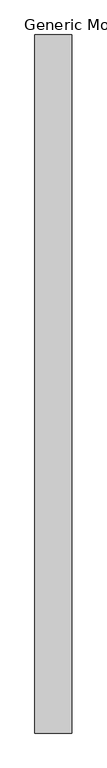
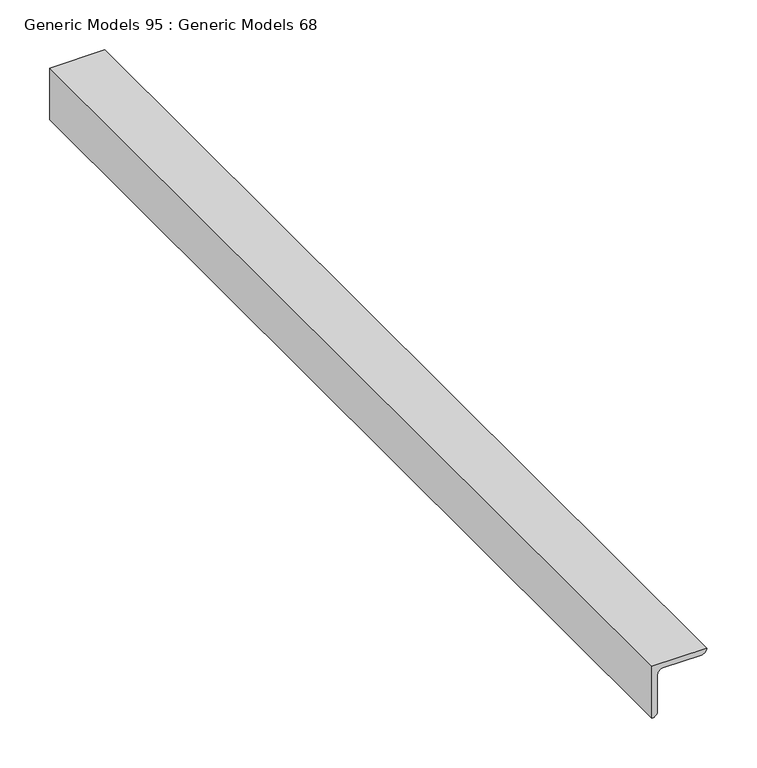
"""IFC4 building model written with IfcOpenShell, lengths in millimetres: proxy geometry, Generic Models 95 : Generic Models 68."""

from ifc_helpers import new_model, si_unit, point, frame, frame_2d, origin, place, context, project, spatial, polyline, circle_curve, trimmed, segment, composite_curve, outline, extrude, source, transform, mapped, element, save


def generic_models_95_generic_models_68_966be8c5(model_context):
    return source(origin(), model_context, "Body", "SweptSolid", [
        extrude(outline(composite_curve([segment(polyline([(266004.6986952, 20536.7616945), (265941.1986952, 20536.7616945)]), True, "CONTINUOUS"), segment(trimmed(circle_curve(frame_2d((265947.5486952, 20536.7616945)), 6.35), [point((265941.1986952, 20536.7616945))], [point((265947.5486952, 20543.1116945))], False, "CARTESIAN"), True, "CONTINUOUS"), segment(polyline([(265947.5486952, 20543.1116945), (265991.9986952, 20543.1116945)]), True, "CONTINUOUS"), segment(trimmed(circle_curve(frame_2d((265991.9986952, 20549.4616945)), 6.35), [point((265991.9986952, 20543.1116945))], [point((265998.3486952, 20549.4616945))], True, "CARTESIAN"), True, "CONTINUOUS"), segment(polyline([(265998.3486952, 20549.4616945), (265998.3486952, 20593.9116945)]), True, "CONTINUOUS"), segment(trimmed(circle_curve(frame_2d((266004.6986952, 20593.9116945)), 6.35), [point((265998.3486952, 20593.9116945))], [point((266004.6986952, 20600.2616945))], False, "CARTESIAN"), True, "CONTINUOUS"), segment(polyline([(266004.6986952, 20600.2616945), (266004.6986952, 20536.7616945)]), True, "CONTINUOUS")], self_intersect=False)), frame((0.0, 20940.7764581, 0.0), z_axis=(0.0, 1.0, 0.0), x_axis=(0.0, 0.0, 1.0)), (0.0, 0.0, 1.0), 1206.5),
    ])


if __name__ == "__main__":
    model = new_model("IFC4")
    model_context = context("Model", 3, world=origin())
    ifc_project = project(units=[si_unit("LENGTHUNIT", "METRE", prefix="MILLI")], contexts=[model_context])
    site = spatial("IfcSite", under=ifc_project)
    building = spatial("IfcBuilding", under=site)
    placement = place(None, origin())
    generic_models_95_generic_models_68_shape = generic_models_95_generic_models_68_966be8c5(model_context)
    element("IfcBuildingElementProxy", 1, Name="Generic Models 95 : Generic Models 68", ObjectType="Generic Models 95 : Generic Models 68", at=placement, inside=building, context=model_context, shape_type="MappedRepresentation", body=[
        mapped(generic_models_95_generic_models_68_shape, transform((0.0, 0.0, 0.0), x_axis=(1.0, 0.0, 0.0), y_axis=(0.0, 1.0, 0.0), z_axis=(0.0, 0.0, 1.0))),
    ])
    save(model, "model.ifc")

# Revit data of these elements
# Element 1 (IfcBuildingElementProxy, "Generic Models 95 : Generic Models 68")
#   Materials on its faces: "CAR DOOR RAIL: GALV. ANGLE L2 1/2 X 2 1/2 X 1/4\" @ 32\" ABOVE GRADE (PARALLEL TO HORTZ. WOOD TRIM)"
# Materials
#   "CAR DOOR RAIL: GALV. ANGLE L2 1/2 X 2 1/2 X 1/4\" @ 32\" ABOVE GRADE (PARALLEL TO HORTZ. WOOD TRIM)": class "Unassigned", colour RGB 211 211 211, transparency 0, Cost = 0
